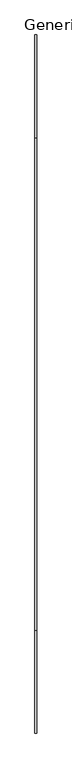
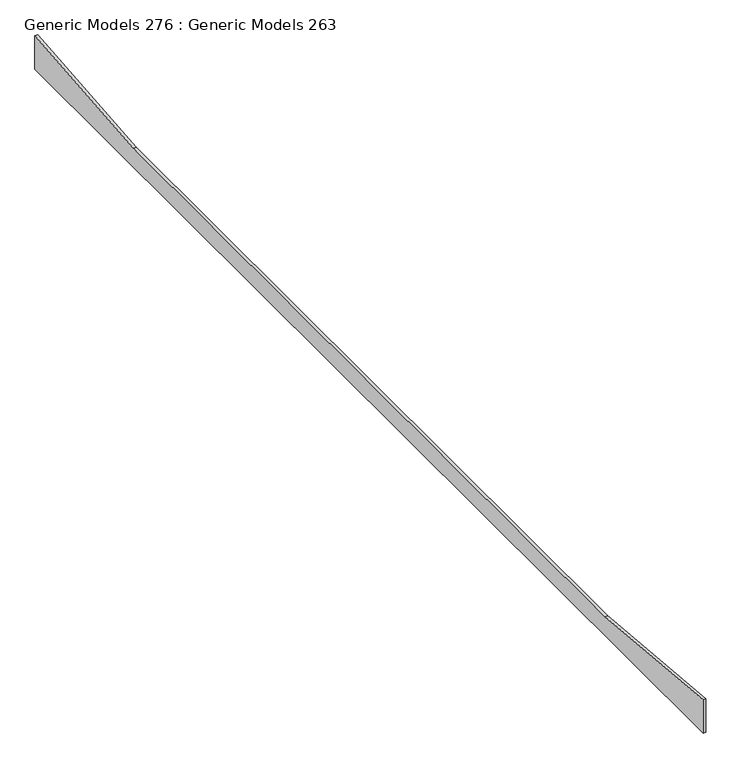
"""IFC4 building model written with IfcOpenShell, lengths in millimetres: proxy geometry, Generic Models 276 : Generic Models 263."""

from ifc_helpers import new_model, si_unit, frame, origin, place, context, project, spatial, polyline, outline, extrude, source, transform, mapped, element, save


def generic_models_276_generic_models_263_4ecf39a9(model_context):
    return source(origin(), model_context, "Body", "SweptSolid", [
        extrude(outline(polyline([(2106.5727422, 2.0699085), (2106.5727422, -314.8198762), (-8256.6272578, -314.8198762), (-8256.6272578, 2.0699085), (-6732.6272578, -137.0198762), (582.5727422, -137.0198762), (2106.5727422, 2.0699085)])), frame((91554.5797726, 0.0, 0.0), z_axis=(1.0, 0.0, 0.0), x_axis=(0.0, 1.0, 0.0)), (0.0, 0.0, 1.0), 25.4),
    ])


if __name__ == "__main__":
    model = new_model("IFC4")
    model_context = context("Model", 3, world=origin())
    ifc_project = project(units=[si_unit("LENGTHUNIT", "METRE", prefix="MILLI")], contexts=[model_context])
    site = spatial("IfcSite", under=ifc_project)
    building = spatial("IfcBuilding", under=site)
    placement = place(None, origin())
    generic_models_276_generic_models_263_shape = generic_models_276_generic_models_263_4ecf39a9(model_context)
    element("IfcBuildingElementProxy", 1, Name="Generic Models 276 : Generic Models 263", ObjectType="Generic Models 276 : Generic Models 263", at=placement, inside=building, context=model_context, shape_type="MappedRepresentation", body=[
        mapped(generic_models_276_generic_models_263_shape, transform((0.0, 0.0, 0.0), x_axis=(1.0, 0.0, 0.0), y_axis=(0.0, 1.0, 0.0), z_axis=(0.0, 0.0, 1.0))),
    ])
    save(model, "model.ifc")

# Revit data of these elements
# Element 1 (IfcBuildingElementProxy, "Generic Models 276 : Generic Models 263")
#   Materials on its faces: "1\" EXPANSION JOINT"
# Materials
#   "1\" EXPANSION JOINT": class "Concrete", colour RGB 197 197 197, transparency 0, Description = "Cast-in-place concrete", Cost = 0
